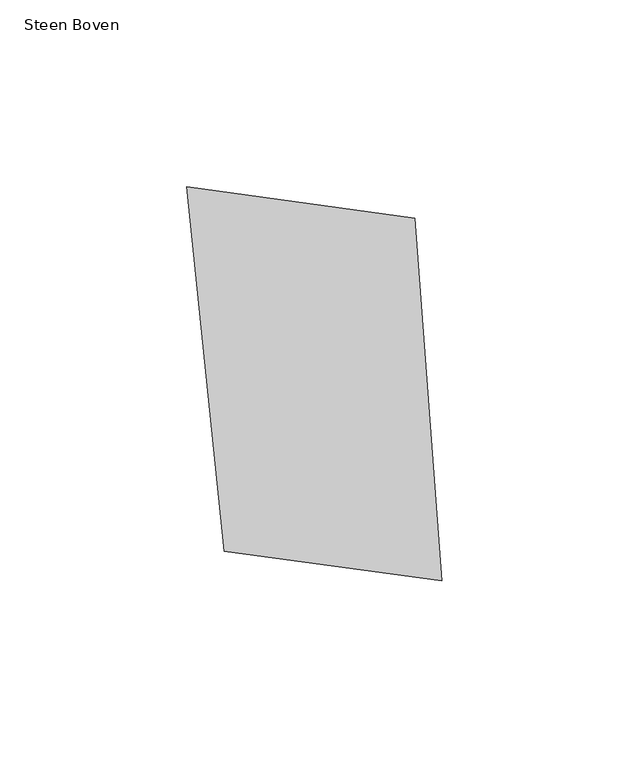
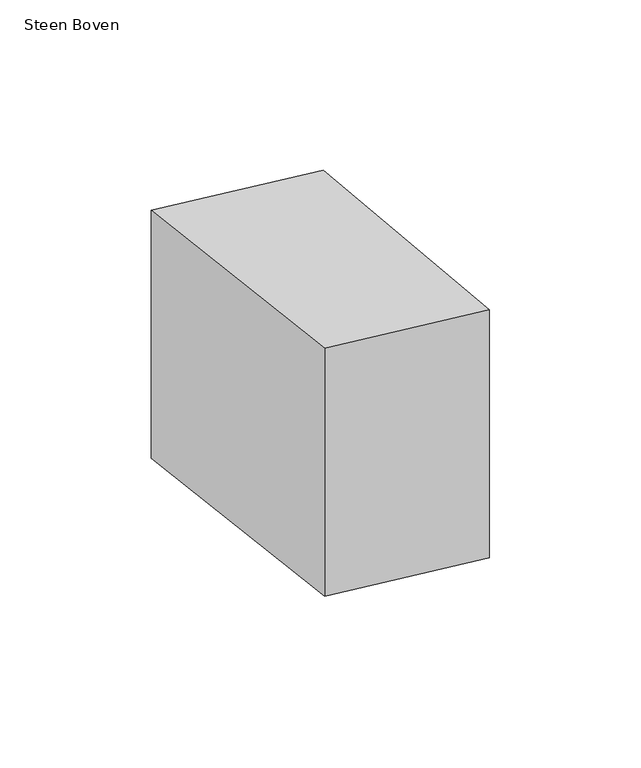
"""IFC4 building model written with IfcOpenShell, lengths in millimetres: proxy geometry, 00_GMA_steen_versie_4 : Steen Boven."""

from ifc_helpers import new_model, si_unit, origin, origin_with_axes, place, context, project, spatial, polyline, outline, extrude, source, transform, mapped, element, save


def steen_boven_cfe30250(model_context):
    return source(origin(), model_context, "Body", "SweptSolid", [
        extrude(outline(polyline([(96.7832521, 120.2686122), (104.0424194, 23.2675536), (45.8803147, 31.2238679), (35.9251654, 128.6210175), (96.7832521, 120.2686122)])), origin_with_axes(), (0.0, 0.0, 1.0), 100.0),
    ])


if __name__ == "__main__":
    model = new_model("IFC4")
    model_context = context("Model", 3, world=origin())
    ifc_project = project(units=[si_unit("LENGTHUNIT", "METRE", prefix="MILLI")], contexts=[model_context])
    site = spatial("IfcSite", under=ifc_project)
    building = spatial("IfcBuilding", under=site)
    placement = place(None, origin())
    steen_boven_shape = steen_boven_cfe30250(model_context)
    element("IfcBuildingElementProxy", 1, Name="00_GMA_steen_versie_4 : Steen Boven", ObjectType="00_GMA_steen_versie_4 : Steen Boven", at=placement, inside=building, context=model_context, shape_type="MappedRepresentation", body=[
        mapped(steen_boven_shape, transform((0.0, 0.0, 0.0), x_axis=(1.0, 0.0, 0.0), y_axis=(0.0, 1.0, 0.0), z_axis=(0.0, 0.0, 1.0))),
    ])
    save(model, "model.ifc")

# Revit data of these elements
# Type "00_GMA_steen_versie_4 : Steen Boven"
#   StootVoegHalfBoven [instance default] = 5 mm
#   StootVoegHalf [instance default] = 5 mm
#   StootVoegBreedteOnder = 10 mm
#   StootVoegBreedteBoven = 10 mm
#   Steendikte = 100 mm
#   LintVoegOnderHalf = 5 mm
#   LintVoegOnder = 10 mm
#   LintVoegBovenHalf = 0 mm
#   LintVoegBoven = 0 mm
#   materiaal = none
#   MateriaalVoeg = none
#   Default Elevation = 0
